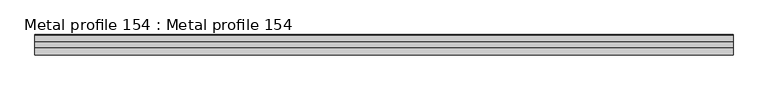
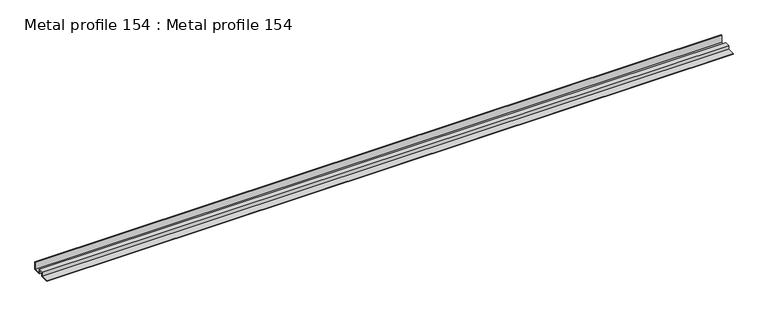
"""IFC4 building model written with IfcOpenShell, lengths in millimetres: proxy geometry, Metal profile 154 : Metal profile 154."""

from ifc_helpers import new_model, si_unit, frame, origin, place, context, project, spatial, polyline, outline, extrude, source, transform, mapped, element, save


def metal_profile_154_metal_profile_154_1631b574(model_context):
    return source(origin(), model_context, "Body", "SweptSolid", [
        extrude(outline(polyline([(10462.1750834, 39401.496), (10439.9500834, 39401.496), (10439.9500834, 39412.926), (10427.2500834, 39412.926), (10427.2500834, 39401.496), (10403.5368994, 39401.496), (10403.5368994, 39402.776), (10425.9700834, 39402.776), (10425.9700834, 39414.206), (10441.2300834, 39414.206), (10441.2300834, 39402.776), (10460.8950834, 39402.776), (10460.8950834, 39425.2967615), (10462.1750834, 39425.2967615), (10462.1750834, 39401.496)])), frame((3694.2883192, 0.0, 0.0), z_axis=(1.0, 0.0, 0.0), x_axis=(0.0, 1.0, 0.0)), (0.0, 0.0, 1.0), 2000.0),
    ])


if __name__ == "__main__":
    model = new_model("IFC4")
    model_context = context("Model", 3, world=origin())
    ifc_project = project(units=[si_unit("LENGTHUNIT", "METRE", prefix="MILLI")], contexts=[model_context])
    site = spatial("IfcSite", under=ifc_project)
    building = spatial("IfcBuilding", under=site)
    placement = place(None, origin())
    metal_profile_154_metal_profile_154_shape = metal_profile_154_metal_profile_154_1631b574(model_context)
    element("IfcBuildingElementProxy", 1, Name="Metal profile 154 : Metal profile 154", ObjectType="Metal profile 154 : Metal profile 154", at=placement, inside=building, context=model_context, shape_type="MappedRepresentation", body=[
        mapped(metal_profile_154_metal_profile_154_shape, transform((0.0, 0.0, 0.0), x_axis=(1.0, 0.0, 0.0), y_axis=(0.0, 1.0, 0.0), z_axis=(0.0, 0.0, 1.0))),
    ])
    save(model, "model.ifc")

# Revit data of these elements
# Type "Metal profile 154 : Metal profile 154"
#   NameOverride = "Metal profile"
# Element 1 (IfcBuildingElementProxy, "Metal profile 154 : Metal profile 154")
#   Materials on its faces: "16 GA. COPPER SOFFIT DRIP SCREED"
# Materials
#   "16 GA. COPPER SOFFIT DRIP SCREED": class "Unassigned", colour RGB 255 217 0, transparency 0
